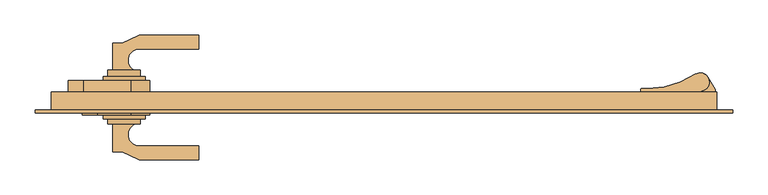
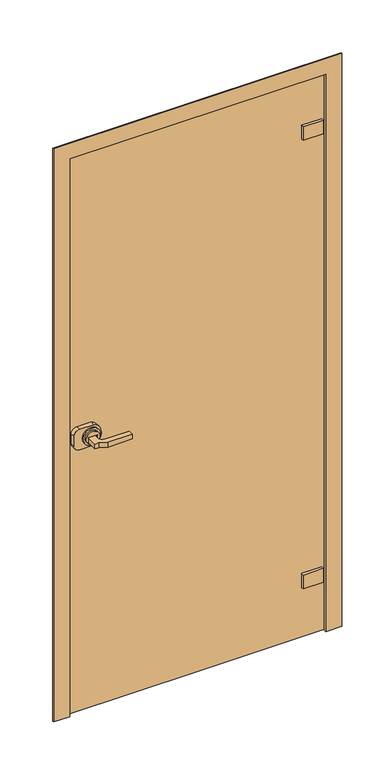
"""IFC4 building model written with IfcOpenShell, lengths in millimetres: door geometry, Doors_Doors_Faraone_Anta : Doors_Doors_Faraone_Anta."""

from ifc_helpers import new_model, si_unit, point, frame, frame_2d, origin, place, context, project, spatial, polyline, circle_curve, trimmed, segment, composite_curve, outline, extrude, faceted_brep, source, transform, mapped, element, save


def door_8e35aac2(model_context):
    return source(origin(), model_context, "Body", "SolidModel", [
        extrude(outline(polyline([(366.2008975, -11.599726), (366.2008975, -1.8997991), (435.9003723, -1.8997991), (435.9003723, -11.599726), (366.2008975, -11.599726)])), frame((0.0, 0.0, 1819.0000277), z_axis=(0.0, 0.0, 1.0), x_axis=(1.0, 0.0, 0.0)), (0.0, 0.0, 1.0), 50.0),
        extrude(outline(composite_curve([segment(trimmed(circle_curve(frame_2d((368.2008824, 17.600054)), 1.9999849), [point((366.2008975, 17.600054))], [point((368.2008824, 19.6000389))], False, "CARTESIAN"), True, "CONTINUOUS"), segment(polyline([(368.2008824, 19.6000389), (376.2008221, 19.6000389)]), True, "CONTINUOUS"), segment(trimmed(circle_curve(frame_2d((374.7862865, 147.5843675)), 127.9921454), [point((376.2008221, 19.6000389))], [point((444.4124725, 40.1870515))], True, "CARTESIAN"), True, "CONTINUOUS"), segment(trimmed(circle_curve(frame_2d((451.200257, 29.0999673)), 12.9999021), [point((444.4124725, 40.1870515))], [point((455.8396194, 16.9560894))], False, "CARTESIAN"), True, "CONTINUOUS"), segment(polyline([(455.8396194, 16.9560894), (436.2003701, 9.6001143), (436.2003701, 8.1001256), (366.2008975, 8.1001256), (366.2008975, 17.600054)]), True, "CONTINUOUS")], self_intersect=False)), frame((0.0, 0.0, 1819.0000277), z_axis=(0.0, 0.0, 1.0), x_axis=(1.0, 0.0, 0.0)), (0.0, 0.0, 1.0), 50.0),
        extrude(outline(composite_curve([segment(polyline([(473.0000928, 18.0609582), (473.0000928, 15.0000736), (451.2037355, 15.0000736), (446.8171202, 16.861276)]), True, "CONTINUOUS"), segment(trimmed(circle_curve(frame_2d((451.200257, 29.0999673)), 12.9999021), [point((446.8171202, 16.861276))], [point((440.8509495, 36.9669419))], False, "CARTESIAN"), True, "CONTINUOUS"), segment(trimmed(circle_curve(frame_2d((451.200257, 29.0999673)), 12.9999021), [point((440.8509495, 36.9669419))], [point((462.2229983, 35.9917471))], False, "CARTESIAN"), True, "CONTINUOUS"), segment(polyline([(462.2229983, 35.9917471), (473.0000928, 18.0609582)]), True, "CONTINUOUS")], self_intersect=False)), frame((0.0, 0.0, 1769.0000277), z_axis=(0.0, 0.0, 1.0), x_axis=(1.0, 0.0, 0.0)), (0.0, 0.0, 1.0), 50.0),
        extrude(outline(polyline([(366.2008975, -11.599726), (366.2008975, -1.8997991), (435.9003723, -1.8997991), (435.9003723, -11.599726), (366.2008975, -11.599726)])), frame((0.0, 0.0, 182.0), z_axis=(0.0, 0.0, 1.0), x_axis=(1.0, 0.0, 0.0)), (0.0, 0.0, 1.0), 50.0),
        extrude(outline(composite_curve([segment(trimmed(circle_curve(frame_2d((368.2008824, 17.600054)), 1.9999849), [point((366.2008975, 17.600054))], [point((368.2008824, 19.6000389))], False, "CARTESIAN"), True, "CONTINUOUS"), segment(polyline([(368.2008824, 19.6000389), (376.2008221, 19.6000389)]), True, "CONTINUOUS"), segment(trimmed(circle_curve(frame_2d((374.7862865, 147.5843675)), 127.9921454), [point((376.2008221, 19.6000389))], [point((444.4124725, 40.1870515))], True, "CARTESIAN"), True, "CONTINUOUS"), segment(trimmed(circle_curve(frame_2d((451.200257, 29.0999673)), 12.9999021), [point((444.4124725, 40.1870515))], [point((455.8396194, 16.9560894))], False, "CARTESIAN"), True, "CONTINUOUS"), segment(polyline([(455.8396194, 16.9560894), (436.2003701, 9.6001143), (436.2003701, 8.1001256), (366.2008975, 8.1001256), (366.2008975, 17.600054)]), True, "CONTINUOUS")], self_intersect=False)), frame((0.0, 0.0, 182.0), z_axis=(0.0, 0.0, 1.0), x_axis=(1.0, 0.0, 0.0)), (0.0, 0.0, 1.0), 50.0),
        extrude(outline(composite_curve([segment(polyline([(473.0000928, 18.0609582), (473.0000928, 15.0000736), (451.2037355, 15.0000736), (446.8171202, 16.861276)]), True, "CONTINUOUS"), segment(trimmed(circle_curve(frame_2d((451.200257, 29.0999673)), 12.9999021), [point((446.8171202, 16.861276))], [point((440.8509495, 36.9669419))], False, "CARTESIAN"), True, "CONTINUOUS"), segment(trimmed(circle_curve(frame_2d((451.200257, 29.0999673)), 12.9999021), [point((440.8509495, 36.9669419))], [point((462.2229983, 35.9917471))], False, "CARTESIAN"), True, "CONTINUOUS"), segment(polyline([(462.2229983, 35.9917471), (473.0000928, 18.0609582)]), True, "CONTINUOUS")], self_intersect=False)), frame((0.0, 0.0, 132.0), z_axis=(0.0, 0.0, 1.0), x_axis=(1.0, 0.0, 0.0)), (0.0, 0.0, 1.0), 50.0),
        extrude(outline(composite_curve([segment(trimmed(circle_curve(frame_2d((1003.2884985, -370.8959538)), 23.0897305), [point((1003.2884985, -393.9856843))], [point((1003.2884985, -347.8062233))], False, "CARTESIAN"), True, "CONTINUOUS"), segment(trimmed(circle_curve(frame_2d((1003.2884985, -370.8959538)), 23.0897305), [point((1003.2884985, -347.8062233))], [point((1003.2884985, -393.9856843))], False, "CARTESIAN"), True, "CONTINUOUS")], self_intersect=False)), frame((0.0, 36.9863146, 0.0), z_axis=(0.0, 1.0, 0.0), x_axis=(0.0, 0.0, 1.0)), (0.0, 0.0, 1.0), 9.3686894),
        extrude(outline(composite_curve([segment(trimmed(circle_curve(frame_2d((987.7717852, -428.4834563)), 22.4105262), [point((983.5880679, -450.5))], [point((965.361259, -428.4834563))], False, "CARTESIAN"), True, "CONTINUOUS"), segment(polyline([(965.361259, -428.4834563), (965.361259, -363.4834563)]), True, "CONTINUOUS"), segment(trimmed(circle_curve(frame_2d((1002.861259, -373.1489886)), 38.7256054), [point((965.361259, -363.4834563))], [point((1039.5100566, -360.6374682))], False, "CARTESIAN"), True, "CONTINUOUS"), segment(polyline([(1039.5100566, -360.6374682), (1039.5100566, -428.4834563)]), True, "CONTINUOUS"), segment(trimmed(circle_curve(frame_2d((1017.0995304, -428.4834563)), 22.4105262), [point((1039.5100566, -428.4834563))], [point((1021.2832478, -450.5))], False, "CARTESIAN"), True, "CONTINUOUS"), segment(polyline([(1021.2832478, -450.5), (983.5880679, -450.5)]), True, "CONTINUOUS")], self_intersect=False)), frame((0.0, 8.1001256, 0.0), z_axis=(0.0, 1.0, 0.0), x_axis=(0.0, 0.0, 1.0)), (0.0, 0.0, 1.0), 23.0652027),
        extrude(outline(composite_curve([segment(trimmed(circle_curve(frame_2d((987.7717852, -428.4834563)), 22.4105262), [point((983.5880679, -450.5))], [point((965.361259, -428.4834563))], False, "CARTESIAN"), True, "CONTINUOUS"), segment(polyline([(965.361259, -428.4834563), (965.361259, -363.4834563)]), True, "CONTINUOUS"), segment(trimmed(circle_curve(frame_2d((1002.861259, -373.1489886)), 38.7256054), [point((965.361259, -363.4834563))], [point((1039.5100566, -360.6374682))], False, "CARTESIAN"), True, "CONTINUOUS"), segment(polyline([(1039.5100566, -360.6374682), (1039.5100566, -428.4834563)]), True, "CONTINUOUS"), segment(trimmed(circle_curve(frame_2d((1017.0995304, -428.4834563)), 22.4105262), [point((1039.5100566, -428.4834563))], [point((1021.2832478, -450.5))], False, "CARTESIAN"), True, "CONTINUOUS"), segment(polyline([(1021.2832478, -450.5), (983.5880679, -450.5)]), True, "CONTINUOUS")], self_intersect=False)), frame((0.0, 8.1001256, 0.0), z_axis=(0.0, 1.0, 0.0), x_axis=(0.0, 0.0, 1.0)), (0.0, 0.0, 1.0), 23.0652027),
        extrude(outline(composite_curve([segment(trimmed(circle_curve(frame_2d((1003.2884985, -370.8959538)), 30.0), [point((1003.2884985, -400.8959538))], [point((1003.2884985, -340.8959538))], False, "CARTESIAN"), True, "CONTINUOUS"), segment(trimmed(circle_curve(frame_2d((1003.2884985, -370.8959538)), 30.0), [point((1003.2884985, -340.8959538))], [point((1003.2884985, -400.8959538))], False, "CARTESIAN"), True, "CONTINUOUS")], self_intersect=False)), frame((0.0, 31.1653283, 0.0), z_axis=(0.0, 1.0, 0.0), x_axis=(0.0, 0.0, 1.0)), (0.0, 0.0, 1.0), 5.8209863),
        extrude(outline(composite_curve([segment(trimmed(circle_curve(frame_2d((987.7717852, -428.4834563)), 22.4105262), [point((983.5880679, -450.5))], [point((965.361259, -428.4834563))], False, "CARTESIAN"), True, "CONTINUOUS"), segment(polyline([(965.361259, -428.4834563), (965.361259, -363.4834563)]), True, "CONTINUOUS"), segment(trimmed(circle_curve(frame_2d((1002.861259, -373.1489886)), 38.7256054), [point((965.361259, -363.4834563))], [point((1039.5100566, -360.6374682))], False, "CARTESIAN"), True, "CONTINUOUS"), segment(polyline([(1039.5100566, -360.6374682), (1039.5100566, -428.4834563)]), True, "CONTINUOUS"), segment(trimmed(circle_curve(frame_2d((1017.0995304, -428.4834563)), 22.4105262), [point((1039.5100566, -428.4834563))], [point((1021.2832478, -450.5))], False, "CARTESIAN"), True, "CONTINUOUS"), segment(polyline([(1021.2832478, -450.5), (983.5880679, -450.5)]), True, "CONTINUOUS")], self_intersect=False)), frame((0.0, 8.1001256, 0.0), z_axis=(0.0, 1.0, 0.0), x_axis=(0.0, 0.0, 1.0)), (0.0, 0.0, 1.0), 23.0652027),
        extrude(outline(composite_curve([segment(trimmed(circle_curve(frame_2d((1003.2884985, -370.8959538)), 23.0897305), [point((1003.2884985, -393.9856843))], [point((1003.2884985, -347.8062233))], False, "CARTESIAN"), True, "CONTINUOUS"), segment(trimmed(circle_curve(frame_2d((1003.2884985, -370.8959538)), 23.0897305), [point((1003.2884985, -347.8062233))], [point((1003.2884985, -393.9856843))], False, "CARTESIAN"), True, "CONTINUOUS")], self_intersect=False)), frame((0.0, 32.1653283, 0.0), z_axis=(0.0, 1.0, 0.0), x_axis=(0.0, 0.0, 1.0)), (0.0, 0.0, 1.0), 14.1896757),
        extrude(outline(composite_curve([segment(trimmed(circle_curve(frame_2d((987.7717852, -428.4834563)), 22.4105262), [point((983.5880679, -450.5))], [point((965.361259, -428.4834563))], False, "CARTESIAN"), True, "CONTINUOUS"), segment(polyline([(965.361259, -428.4834563), (965.361259, -363.4834563)]), True, "CONTINUOUS"), segment(trimmed(circle_curve(frame_2d((1002.861259, -373.1489886)), 38.7256054), [point((965.361259, -363.4834563))], [point((1039.5100566, -360.6374682))], False, "CARTESIAN"), True, "CONTINUOUS"), segment(polyline([(1039.5100566, -360.6374682), (1039.5100566, -428.4834563)]), True, "CONTINUOUS"), segment(trimmed(circle_curve(frame_2d((1017.0995304, -428.4834563)), 22.4105262), [point((1039.5100566, -428.4834563))], [point((1021.2832478, -450.5))], False, "CARTESIAN"), True, "CONTINUOUS"), segment(polyline([(1021.2832478, -450.5), (983.5880679, -450.5)]), True, "CONTINUOUS")], self_intersect=False)), frame((0.0, 8.1001256, 0.0), z_axis=(0.0, 1.0, 0.0), x_axis=(0.0, 0.0, 1.0)), (0.0, 0.0, 1.0), 23.0652027),
        extrude(outline(composite_curve([segment(trimmed(circle_curve(frame_2d((987.7717852, -428.4834563)), 22.4105262), [point((983.5880679, -450.5))], [point((965.361259, -428.4834563))], False, "CARTESIAN"), True, "CONTINUOUS"), segment(polyline([(965.361259, -428.4834563), (965.361259, -363.4834563)]), True, "CONTINUOUS"), segment(trimmed(circle_curve(frame_2d((1002.861259, -373.1489886)), 38.7256054), [point((965.361259, -363.4834563))], [point((1039.5100566, -360.6374682))], False, "CARTESIAN"), True, "CONTINUOUS"), segment(polyline([(1039.5100566, -360.6374682), (1039.5100566, -428.4834563)]), True, "CONTINUOUS"), segment(trimmed(circle_curve(frame_2d((1017.0995304, -428.4834563)), 22.4105262), [point((1039.5100566, -428.4834563))], [point((1021.2832478, -450.5))], False, "CARTESIAN"), True, "CONTINUOUS"), segment(polyline([(1021.2832478, -450.5), (983.5880679, -450.5)]), True, "CONTINUOUS")], self_intersect=False)), frame((0.0, 8.1001256, 0.0), z_axis=(0.0, 1.0, 0.0), x_axis=(0.0, 0.0, 1.0)), (0.0, 0.0, 1.0), 23.0652027),
        extrude(outline(composite_curve([segment(polyline([(-387.3305508, 84.9663543), (-373.6484437, 84.9663543), (-349.204395, 96.3648014), (-264.204395, 96.3648014), (-264.204395, 76.3648014), (-349.204395, 76.3648014)]), True, "CONTINUOUS"), segment(trimmed(circle_curve(frame_2d((-349.204395, 60.2485058)), 16.1162956), [point((-349.204395, 76.3648014))], [point((-357.3717442, 46.355004))], True, "CARTESIAN"), True, "CONTINUOUS"), segment(polyline([(-357.3717442, 46.355004), (-387.3305508, 46.355004), (-387.3305508, 84.9663543)]), True, "CONTINUOUS")], self_intersect=False)), frame((0.0, 0.0, 992.5658854), z_axis=(0.0, 0.0, 1.0), x_axis=(1.0, 0.0, 0.0)), (0.0, 0.0, 1.0), 16.6938628),
        extrude(outline(composite_curve([segment(trimmed(circle_curve(frame_2d((987.7717852, -428.4834563)), 22.4105262), [point((983.5880679, -450.5))], [point((965.361259, -428.4834563))], False, "CARTESIAN"), True, "CONTINUOUS"), segment(polyline([(965.361259, -428.4834563), (965.361259, -363.4834563)]), True, "CONTINUOUS"), segment(trimmed(circle_curve(frame_2d((1002.861259, -373.1489886)), 38.7256054), [point((965.361259, -363.4834563))], [point((1039.5100566, -360.6374682))], False, "CARTESIAN"), True, "CONTINUOUS"), segment(polyline([(1039.5100566, -360.6374682), (1039.5100566, -428.4834563)]), True, "CONTINUOUS"), segment(trimmed(circle_curve(frame_2d((1017.0995304, -428.4834563)), 22.4105262), [point((1039.5100566, -428.4834563))], [point((1021.2832478, -450.5))], False, "CARTESIAN"), True, "CONTINUOUS"), segment(polyline([(1021.2832478, -450.5), (983.5880679, -450.5)]), True, "CONTINUOUS")], self_intersect=False)), frame((0.0, 8.1001256, 0.0), z_axis=(0.0, 1.0, 0.0), x_axis=(0.0, 0.0, 1.0)), (0.0, 0.0, 1.0), 23.0652027),
        extrude(outline(composite_curve([segment(trimmed(circle_curve(frame_2d((1003.2884985, -370.8959538)), 23.0897305), [point((1003.2884985, -393.9856843))], [point((1003.2884985, -347.8062233))], False, "CARTESIAN"), True, "CONTINUOUS"), segment(trimmed(circle_curve(frame_2d((1003.2884985, -370.8959538)), 23.0897305), [point((1003.2884985, -347.8062233))], [point((1003.2884985, -393.9856843))], False, "CARTESIAN"), True, "CONTINUOUS")], self_intersect=False)), frame((0.0, -30.8998744, 0.0), z_axis=(0.0, 1.0, 0.0), x_axis=(0.0, 0.0, 1.0)), (0.0, 0.0, 1.0), 7.0),
        extrude(outline(composite_curve([segment(trimmed(circle_curve(frame_2d((987.7717852, -408.4834563)), 22.4105262), [point((983.5880679, -430.5))], [point((965.361259, -408.4834563))], False, "CARTESIAN"), True, "CONTINUOUS"), segment(polyline([(965.361259, -408.4834563), (965.361259, -363.4834563)]), True, "CONTINUOUS"), segment(trimmed(circle_curve(frame_2d((1002.861259, -373.1489886)), 38.7256054), [point((965.361259, -363.4834563))], [point((1039.5100566, -360.6374682))], False, "CARTESIAN"), True, "CONTINUOUS"), segment(polyline([(1039.5100566, -360.6374682), (1039.5100566, -408.4834563)]), True, "CONTINUOUS"), segment(trimmed(circle_curve(frame_2d((1017.0995304, -408.4834563)), 22.4105262), [point((1039.5100566, -408.4834563))], [point((1021.2832478, -430.5))], False, "CARTESIAN"), True, "CONTINUOUS"), segment(polyline([(1021.2832478, -430.5), (983.5880679, -430.5)]), True, "CONTINUOUS")], self_intersect=False)), frame((0.0, -17.8998744, 0.0), z_axis=(0.0, 1.0, 0.0), x_axis=(0.0, 0.0, 1.0)), (0.0, 0.0, 1.0), 16.0),
        extrude(outline(composite_curve([segment(polyline([(-387.3305508, -70.762087), (-387.3305508, -30.8998744), (-354.7164928, -30.8998744)]), True, "CONTINUOUS"), segment(trimmed(circle_curve(frame_2d((-349.204395, -46.0442385)), 16.1162956), [point((-354.7164928, -30.8998744))], [point((-349.204395, -62.1605341))], True, "CARTESIAN"), True, "CONTINUOUS"), segment(polyline([(-349.204395, -62.1605341), (-264.204395, -62.1605341), (-264.204395, -82.1605341), (-349.204395, -82.1605341), (-373.6484437, -70.762087), (-387.3305508, -70.762087)]), True, "CONTINUOUS")], self_intersect=False)), frame((0.0, 0.0, 992.5658854), z_axis=(0.0, 0.0, 1.0), x_axis=(1.0, 0.0, 0.0)), (0.0, 0.0, 1.0), 16.6938628),
        extrude(outline(composite_curve([segment(trimmed(circle_curve(frame_2d((1003.2884985, -370.8959538)), 30.0), [point((1003.2884985, -400.8959538))], [point((1003.2884985, -340.8959538))], False, "CARTESIAN"), True, "CONTINUOUS"), segment(trimmed(circle_curve(frame_2d((1003.2884985, -370.8959538)), 30.0), [point((1003.2884985, -340.8959538))], [point((1003.2884985, -400.8959538))], False, "CARTESIAN"), True, "CONTINUOUS")], self_intersect=False)), frame((0.0, -23.8998744, 0.0), z_axis=(0.0, 1.0, 0.0), x_axis=(0.0, 0.0, 1.0)), (0.0, 0.0, 1.0), 6.0),
        faceted_brep([(-442.0002625, -14.999774, 0.0), (-497.9998241, -14.999774, 0.0), (-497.9998241, -11.2997382, 0.0), (-488.6999352, -11.2997382, 0.0), (-488.6999352, -12.9997254, 0.0), (-475.0, -12.9997254, 0.0), (-475.0, 15.0, 0.0), (-457.0001619, 15.0, 0.0), (-457.0001619, -5.9998078, 0.0), (-442.0002625, -5.9998078, 0.0), (-442.0002625, -5.9998078, 2037.0002901), (-442.0002625, -14.999774, 2037.0002901), (-457.0001619, -5.9998078, 2052.0001896), (457.0001619, -5.9998078, 2052.0001896), (457.0001619, -5.9998078, 0.0), (442.0002625, -5.9998078, 0.0), (442.0002625, -5.9998078, 2037.0002901), (-457.0001619, 15.0, 2052.0001896), (-475.0, 15.0, 2070.0000277), (475.0, 15.0, 2070.0000277), (475.0, 15.0, 0.0), (457.0001619, 15.0, 0.0), (457.0001619, 15.0, 2052.0001896), (-475.0, -12.9997254, 2070.0000277), (-488.6999352, -12.9997254, 2083.6999629), (488.6999352, -12.9997254, 2083.6999629), (488.6999352, -12.9997254, 0.0), (475.0, -12.9997254, 0.0), (475.0, -12.9997254, 2070.0000277), (-488.6999352, -11.2997382, 2083.6999629), (-497.9998241, -11.2997382, 2092.9998518), (497.9998241, -11.2997382, 2092.9998518), (497.9998241, -11.2997382, 0.0), (488.6999352, -11.2997382, 0.0), (488.6999352, -11.2997382, 2083.6999629), (-497.9998241, -14.999774, 2092.9998518), (442.0002625, -14.999774, 2037.0002901), (442.0002625, -14.999774, 0.0), (497.9998241, -14.999774, 0.0), (497.9998241, -14.999774, 2092.9998518)], [[[0, 1, 2, 3, 4, 5, 6, 7, 8, 9]], [[9, 10, 11, 0]], [[8, 12, 13, 14, 15, 16, 10, 9]], [[7, 17, 12, 8]], [[6, 18, 19, 20, 21, 22, 17, 7]], [[5, 23, 18, 6]], [[4, 24, 25, 26, 27, 28, 23, 5]], [[3, 29, 24, 4]], [[2, 30, 31, 32, 33, 34, 29, 3]], [[1, 35, 30, 2]], [[0, 11, 36, 37, 38, 39, 35, 1]], [[16, 15, 37, 36]], [[37, 15, 14, 21, 20, 27, 26, 33, 32, 38]], [[22, 21, 14, 13]], [[28, 27, 20, 19]], [[34, 33, 26, 25]], [[39, 38, 32, 31]], [[10, 16, 36, 11]], [[17, 22, 13, 12]], [[23, 28, 19, 18]], [[29, 34, 25, 24]], [[35, 39, 31, 30]]]),
        extrude(outline(polyline([(0.0, -450.5), (0.0, 9.5), (0.0, 450.5), (2043.9998511, 450.5), (2043.9998511, -450.5), (0.0, -450.5)])), frame((0.0, -1.8998744, 0.0), z_axis=(0.0, 1.0, 0.0), x_axis=(0.0, 0.0, 1.0)), (0.0, 0.0, 1.0), 10.0),
    ])


if __name__ == "__main__":
    model = new_model("IFC4")
    model_context = context("Model", 3, world=origin())
    ifc_project = project(units=[si_unit("LENGTHUNIT", "METRE", prefix="MILLI")], contexts=[model_context])
    site = spatial("IfcSite", under=ifc_project)
    building = spatial("IfcBuilding", under=site)
    placement = place(None, origin())
    door_shape = door_8e35aac2(model_context)
    element("IfcDoor", 1, ObjectType="Doors_Doors_Faraone_Anta : Doors_Doors_Faraone_Anta", at=placement, inside=building, context=model_context, shape_type="MappedRepresentation", body=[
        mapped(door_shape, transform((0.0, 0.0, 0.0), x_axis=(1.0, 0.0, 0.0), y_axis=(0.0, 1.0, 0.0), z_axis=(0.0, 0.0, 1.0))),
    ])
    save(model, "model.ifc")

# Revit data of these elements
# Type "Doors_Doors_Faraone_Anta : Doors_Doors_Faraone_Anta"
#   Type Mark = "58"
#   URL = "https://faraone.it/en/"
#   Product data url = ""
#   Product Guid = ""
#   Model = "Spazio_Anta"
#   Manufacturer = "Faraone"
#   Keynote = "08110"
#   Assembly Code = "C1020100"
#   Analytic Construction = "<None>"
#   Width [instance default] = 1104.999 mm
#   Height [instance default] = 2700 mm
#   Handle Height = 1000 mm
#   Thickness = 11 mm
#   Glass Width [instance default] = 1055.999 mm
#   Middle Hinge [instance default] = yes
#   Edition number = 1
#   Define Thermal Properties by = 1
#   Interior Material = Glass - Faraone - Transparent
#   Handle Type = element 507032
#   Exterior Material = Aluminium - Faraone - Silver
#   Function = (empty or 0)
# Element 1 (IfcDoor, "Doors_Doors_Faraone_Anta : Doors_Doors_Faraone_Anta")
#   Width = 950 mm
#   Height = 2070 mm
#   Glass Width = 901 mm
#   Middle Hinge = no
#   Materials on its faces: "Aluminium - Faraone - Silver", "Glass - Faraone - Transparent"
# Materials
#   "Glass - Faraone - Transparent": class "Glass", colour RGB 0 128 192, transparency 0.9, Description = "Soda Lime Glass", Cost = 0
#   "Aluminium - Faraone - Silver": class "Metal", colour RGB 244 244 244, transparency 0, Description = "Metal - Faraone - Aluminium", Cost = 0
